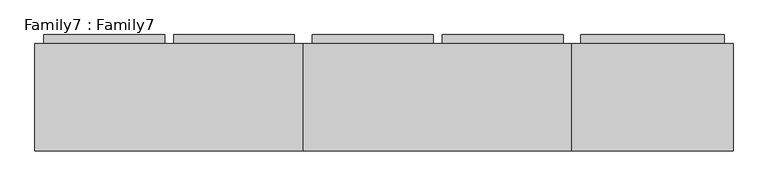
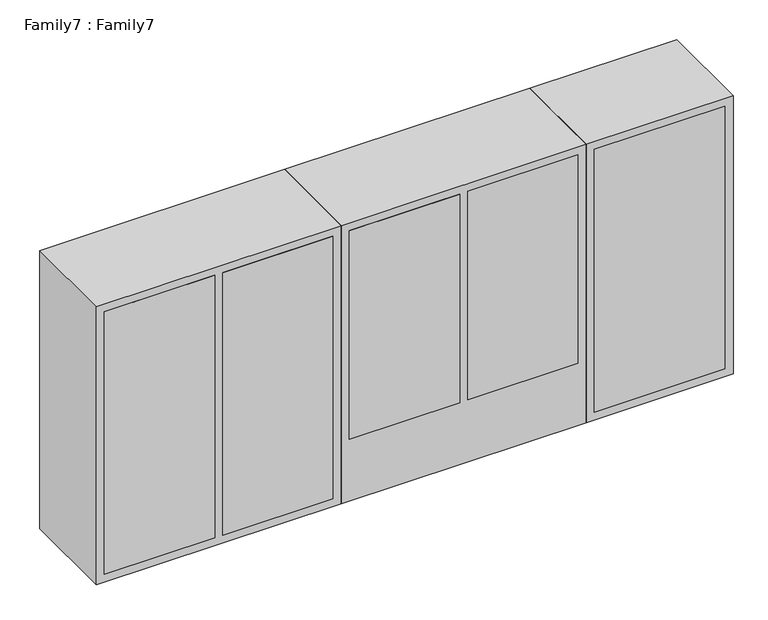
"""IFC4 building model written with IfcOpenShell, lengths in millimetres: proxy geometry, Family7 : Family7."""

from ifc_helpers import new_model, si_unit, frame, origin, place, context, project, spatial, polyline, outline, extrude, source, transform, mapped, element, save


def family7_family7_1379c099(model_context):
    return source(origin(), model_context, "Body", "SweptSolid", [
        extrude(outline(polyline([(1168.4, 381.0), (1574.8, 381.0), (1574.8, 50.8), (1168.4, 50.8), (1168.4, 381.0)])), frame((0.0, 0.0, 1727.1133048), z_axis=(0.0, 0.0, 1.0), x_axis=(1.0, 0.0, 0.0)), (0.0, 0.0, 1.0), 863.6),
        extrude(outline(polyline([(1143.0, 355.6), (1600.2, 355.6), (1600.2, 50.8), (1143.0, 50.8), (1143.0, 355.6)])), frame((0.0, 0.0, 1701.7133048), z_axis=(0.0, 0.0, 1.0), x_axis=(1.0, 0.0, 0.0)), (0.0, 0.0, 1.0), 914.4),
        extrude(outline(polyline([(774.7, 381.0), (1117.6, 381.0), (1117.6, 50.8), (774.7, 50.8), (774.7, 381.0)])), frame((0.0, 0.0, 1904.9133048), z_axis=(0.0, 0.0, 1.0), x_axis=(1.0, 0.0, 0.0)), (0.0, 0.0, 1.0), 685.8),
        extrude(outline(polyline([(406.4, 381.0), (749.3, 381.0), (749.3, 50.8), (406.4, 50.8), (406.4, 381.0)])), frame((0.0, 0.0, 1904.9133048), z_axis=(0.0, 0.0, 1.0), x_axis=(1.0, 0.0, 0.0)), (0.0, 0.0, 1.0), 685.8),
        extrude(outline(polyline([(381.0, 355.6), (1143.0, 355.6), (1143.0, 50.8), (381.0, 50.8), (381.0, 355.6)])), frame((0.0, 0.0, 1701.7133048), z_axis=(0.0, 0.0, 1.0), x_axis=(1.0, 0.0, 0.0)), (0.0, 0.0, 1.0), 914.4),
        extrude(outline(polyline([(12.7, 381.0), (355.6, 381.0), (355.6, 50.8), (12.7, 50.8), (12.7, 381.0)])), frame((0.0, 0.0, 1727.1133048), z_axis=(0.0, 0.0, 1.0), x_axis=(1.0, 0.0, 0.0)), (0.0, 0.0, 1.0), 863.6),
        extrude(outline(polyline([(-355.6, 381.0), (-12.7, 381.0), (-12.7, 50.8), (-355.6, 50.8), (-355.6, 381.0)])), frame((0.0, 0.0, 1727.1133048), z_axis=(0.0, 0.0, 1.0), x_axis=(1.0, 0.0, 0.0)), (0.0, 0.0, 1.0), 863.6),
        extrude(outline(polyline([(-381.0, 355.6), (381.0, 355.6), (381.0, 50.8), (-381.0, 50.8), (-381.0, 355.6)])), frame((0.0, 0.0, 1701.7133048), z_axis=(0.0, 0.0, 1.0), x_axis=(1.0, 0.0, 0.0)), (0.0, 0.0, 1.0), 914.4),
    ])


if __name__ == "__main__":
    model = new_model("IFC4")
    model_context = context("Model", 3, world=origin())
    ifc_project = project(units=[si_unit("LENGTHUNIT", "METRE", prefix="MILLI")], contexts=[model_context])
    site = spatial("IfcSite", under=ifc_project)
    building = spatial("IfcBuilding", under=site)
    placement = place(None, origin())
    family7_family7_shape = family7_family7_1379c099(model_context)
    element("IfcBuildingElementProxy", 1, Name="Family7 : Family7", ObjectType="Family7 : Family7", at=placement, inside=building, context=model_context, shape_type="MappedRepresentation", body=[
        mapped(family7_family7_shape, transform((0.0, 0.0, 0.0), x_axis=(1.0, 0.0, 0.0), y_axis=(0.0, 1.0, 0.0), z_axis=(0.0, 0.0, 1.0))),
    ])
    save(model, "model.ifc")

# Revit data of these elements
# Type "Family7 : Family7"
#   strip spacing = 0' - 1"
#   drawer width = 1' - 3"
#   drawer depth = 1' - 1"
#   cabinet depth = 1' - 0"
#   Default Elevation = 0
